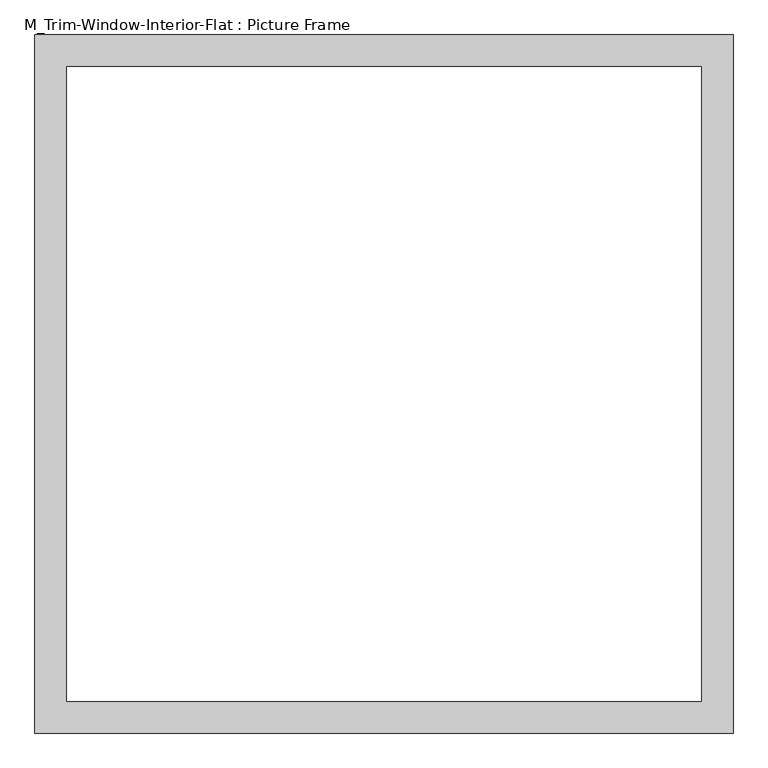
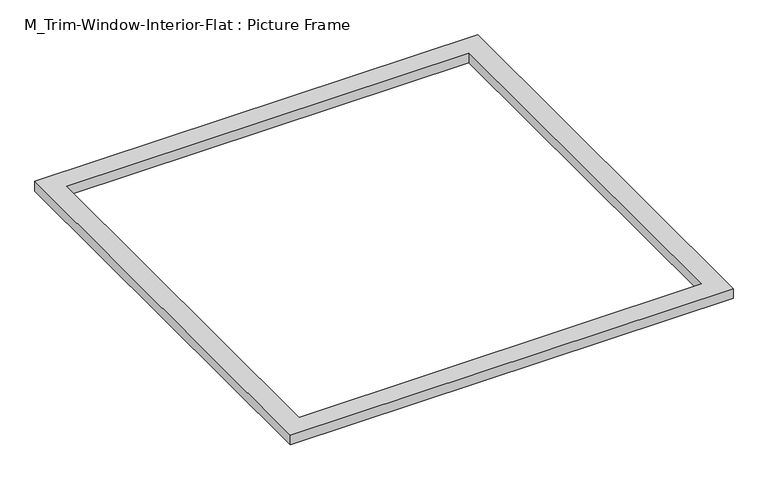
"""IFC4 building model written with IfcOpenShell, lengths in millimetres: proxy geometry, M_Trim-Window-Interior-Flat : Picture Frame."""

from ifc_helpers import new_model, si_unit, origin, origin_with_axes, place, context, project, spatial, polyline, outline, extrude, source, transform, mapped, element, save


def m_trim_window_interior_flat_picture_frame_a73cd484(model_context):
    return source(origin(), model_context, "Body", "SweptSolid", [
        extrude(outline(polyline([(656.9, 47.3), (656.9, -1266.5), (-656.9, -1266.5), (-656.9, 47.3), (656.9, 47.3)]), holes=[polyline([(596.9, -12.7), (-596.9, -12.7), (-596.9, -1206.5), (596.9, -1206.5), (596.9, -12.7)])]), origin_with_axes(), (0.0, 0.0, 1.0), 30.0),
    ])


if __name__ == "__main__":
    model = new_model("IFC4")
    model_context = context("Model", 3, world=origin())
    ifc_project = project(units=[si_unit("LENGTHUNIT", "METRE", prefix="MILLI")], contexts=[model_context])
    site = spatial("IfcSite", under=ifc_project)
    building = spatial("IfcBuilding", under=site)
    placement = place(None, origin())
    m_trim_window_interior_flat_picture_frame_shape = m_trim_window_interior_flat_picture_frame_a73cd484(model_context)
    element("IfcBuildingElementProxy", 1, Name="M_Trim-Window-Interior-Flat : Picture Frame", ObjectType="M_Trim-Window-Interior-Flat : Picture Frame", at=placement, inside=building, context=model_context, shape_type="MappedRepresentation", body=[
        mapped(m_trim_window_interior_flat_picture_frame_shape, transform((0.0, 0.0, 0.0), x_axis=(1.0, 0.0, 0.0), y_axis=(0.0, 1.0, 0.0), z_axis=(0.0, 0.0, 1.0))),
    ])
    save(model, "model.ifc")

# Revit data of these elements
# Type "M_Trim-Window-Interior-Flat : Picture Frame"
#   Trim Thickness_Picture Frame = 0' - 1.1811"
#   Trim Width = 0' - 2.3622"
#   Trim Thickness_with Sill = 0' - 0.7874"
#   Sill Thickness = 0' - 1.1811"
#   Opening Width [instance default] = 1' - 11.62205"
#   Opening Height [instance default] = 2' - 11.43307"
#   Default Elevation = 3' - 11.24409"
#   Sill = no
#   Picture Frame = yes
#   Trim Material [instance default] = none
# Element 1 (IfcBuildingElementProxy, "M_Trim-Window-Interior-Flat : Picture Frame")
#   Opening Width = 4' - 0"
#   Opening Height = 4' - 0"
#   Trim Material = Wood - Stained
#   Materials on its faces: "Wood - Stained"
# Materials
#   "Wood - Stained": class "Wood", colour RGB 224 178 126, transparency 0, Cost = 0
